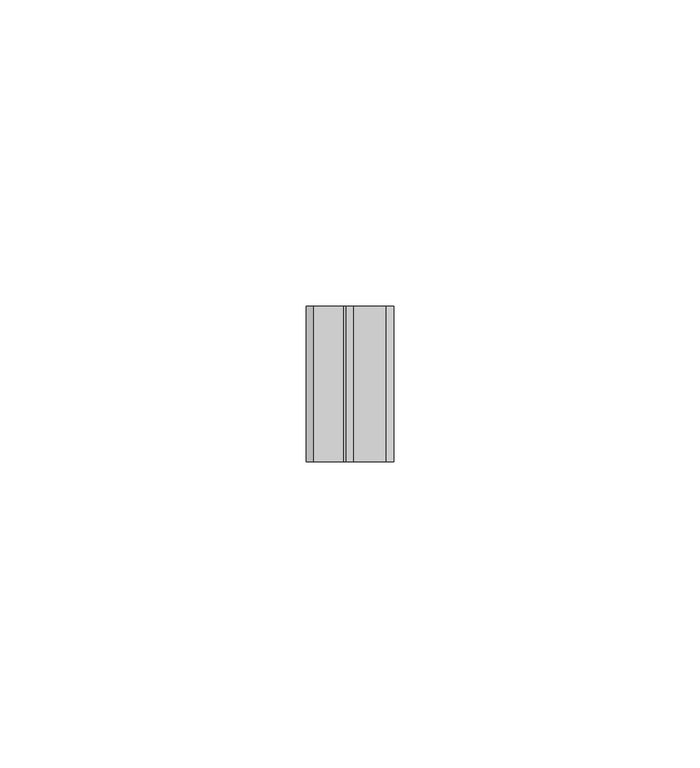
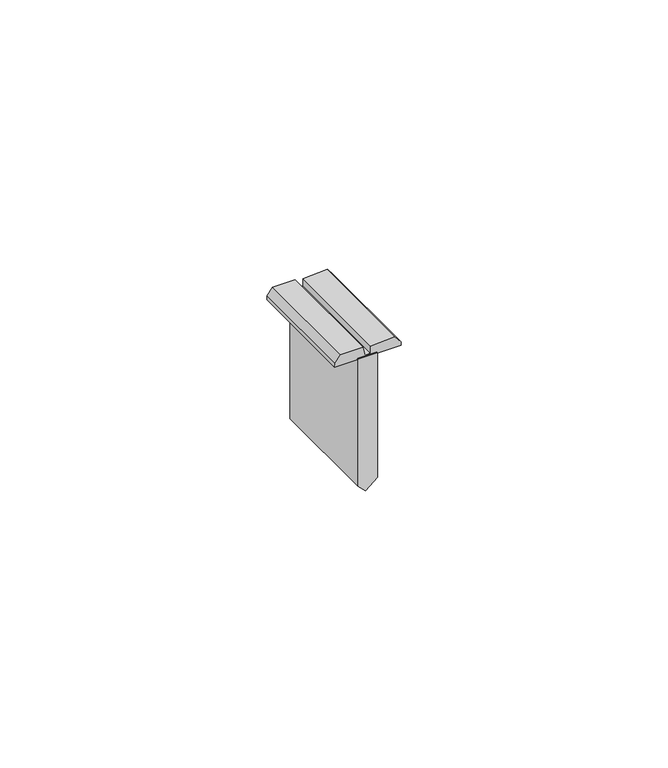
"""IFC4 building model written with IfcOpenShell, lengths in millimetres: proxy geometry, FASTENER005 5969 : FASTENER005 5969."""

import ifcopenshell
import ifcopenshell.guid

model = None  # the IFC model being written
_history = None  # IfcOwnerHistory: only IFC2X3 demands one
_inside = {}  # id of a spatial element -> (the spatial element, [elements in it])
_under = {}  # id of a project, library or spatial element -> (it, [spatial elements below it])
_declared = {}  # id of a project -> (the project, [libraries it declares])
_typed = {}  # id of a type object -> (the type object, [elements of that type])
_made_of = {}  # id of a material, layer set ... -> (it, [elements and type objects made of it])


def new_model(schema):
    """Start an empty IFC model of exactly this schema.

    Asked for "IFC4X3", IfcOpenShell would pick the latest addendum, in which some entities
    have other attributes; the version numbers below select the first issue.
    IFC2X3 requires an IfcOwnerHistory on every rooted entity: one is made here for all.
    """
    global model, _history
    if schema == "IFC4X3":
        model = ifcopenshell.file(schema_version=(4, 3, 0, 0))
    else:
        model = ifcopenshell.file(schema=schema)
    _inside.clear()
    _under.clear()
    _declared.clear()
    _typed.clear()
    _made_of.clear()
    _history = None
    if model.schema == "IFC2X3":
        org = make("IfcOrganization", Name="unknown")
        user = make(
            "IfcPersonAndOrganization",
            ThePerson=make("IfcPerson", FamilyName="unknown"),
            TheOrganization=org,
        )
        app = make(
            "IfcApplication",
            ApplicationDeveloper=org,
            Version="unknown",
            ApplicationFullName="unknown",
            ApplicationIdentifier="unknown",
        )
        _history = make(
            "IfcOwnerHistory",
            OwningUser=user,
            OwningApplication=app,
            ChangeAction="ADDED",
            CreationDate=0,
        )
    return model


def make(cls, **values):
    """One entity of the class cls with the attributes given. An attribute that is None is left unset."""
    return model.create_entity(
        cls, **{name: value for name, value in values.items() if value is not None}
    )


def rooted(cls, **values):
    """An entity with a GlobalId (a new one), such as an element, a storey or a relation."""
    return make(cls, GlobalId=ifcopenshell.guid.new(), OwnerHistory=_history, **values)


def si_unit(unit_type, name, prefix=None):
    """IfcSIUnit, for example si_unit("LENGTHUNIT", "METRE", prefix="MILLI")."""
    return make("IfcSIUnit", UnitType=unit_type, Prefix=prefix, Name=name)


def assignment(units):
    """IfcUnitAssignment: the units of a project."""
    return None if units is None else make("IfcUnitAssignment", Units=units)


def point(xyz):
    """IfcCartesianPoint."""
    return None if xyz is None else make("IfcCartesianPoint", Coordinates=xyz)


def direction(xyz):
    """IfcDirection."""
    return None if xyz is None else make("IfcDirection", DirectionRatios=xyz)


def frame(location, z_axis=None, x_axis=None):
    """IfcAxis2Placement3D, a coordinate frame: its origin and axes. An axis left out is left unset."""
    return make(
        "IfcAxis2Placement3D",
        Location=point(location),
        Axis=direction(z_axis),
        RefDirection=direction(x_axis),
    )


def origin():
    """The frame at (0, 0, 0) with its axes left unset."""
    return frame((0.0, 0.0, 0.0))


def place(relative_to, where):
    """IfcLocalPlacement: puts the frame where relative to a parent placement (None: the world)."""
    return make(
        "IfcLocalPlacement", PlacementRelTo=relative_to, RelativePlacement=where
    )


def context(
    kind, dimensions, precision=None, world=None, true_north=None, identifier=None
):
    """IfcGeometricRepresentationContext, for example the 3D "Model" context."""
    return make(
        "IfcGeometricRepresentationContext",
        ContextIdentifier=identifier,
        ContextType=kind,
        CoordinateSpaceDimension=dimensions,
        Precision=precision,
        WorldCoordinateSystem=world,
        TrueNorth=true_north,
    )


def project(units=None, contexts=None):
    """IfcProject with its units and contexts."""
    return rooted(
        "IfcProject",
        Name="project",
        RepresentationContexts=contexts,
        UnitsInContext=assignment(units),
    )


def spatial(cls, under=None, at=None, **own):
    """A site, building, storey or space (cls), placed at a placement, below another one or the project."""
    s = rooted(cls, ObjectPlacement=at, **own)
    if under is not None:
        _under.setdefault(under.id(), (under, []))[1].append(s)
    return s


def polyline(points):
    """IfcPolyline through the points."""
    return make("IfcPolyline", Points=[point(p) for p in points])


def outline(outer, holes=None, kind="AREA"):
    """IfcArbitraryClosedProfileDef: a profile drawn as a closed curve; with holes, ...WithVoids."""
    if holes is None:
        return make("IfcArbitraryClosedProfileDef", ProfileType=kind, OuterCurve=outer)
    return make(
        "IfcArbitraryProfileDefWithVoids",
        ProfileType=kind,
        OuterCurve=outer,
        InnerCurves=holes,
    )


def extrude(swept, where, along, depth):
    """IfcExtrudedAreaSolid: the profile swept, set in the frame where, extruded along a direction by depth."""
    return make(
        "IfcExtrudedAreaSolid",
        SweptArea=swept,
        Position=where,
        ExtrudedDirection=direction(along),
        Depth=depth,
    )


def shape(context_of_items, identifier, shape_type, items):
    """IfcShapeRepresentation: the items that make up one representation, for example the "Body"."""
    return make(
        "IfcShapeRepresentation",
        ContextOfItems=context_of_items,
        RepresentationIdentifier=identifier,
        RepresentationType=shape_type,
        Items=items,
    )


def source(mapping_origin, context_of_items, identifier, shape_type, items):
    """IfcRepresentationMap: a shape defined once, which mapped items show again and again."""
    return make(
        "IfcRepresentationMap",
        MappingOrigin=mapping_origin,
        MappedRepresentation=shape(context_of_items, identifier, shape_type, items),
    )


def transform(
    local_origin,
    x_axis=None,
    y_axis=None,
    z_axis=None,
    scale=None,
    scale2=None,
    scale3=None,
    uniform=True,
):
    """IfcCartesianTransformationOperator3D, or its non-uniform kind. x_axis, y_axis, z_axis: its Axis1, 2, 3."""
    if uniform:
        return make(
            "IfcCartesianTransformationOperator3D",
            Axis1=direction(x_axis),
            Axis2=direction(y_axis),
            LocalOrigin=point(local_origin),
            Scale=scale,
            Axis3=direction(z_axis),
        )
    return make(
        "IfcCartesianTransformationOperator3DnonUniform",
        Axis1=direction(x_axis),
        Axis2=direction(y_axis),
        LocalOrigin=point(local_origin),
        Scale=scale,
        Axis3=direction(z_axis),
        Scale2=scale2,
        Scale3=scale3,
    )


def mapped(mapping_source, mapping_target):
    """IfcMappedItem: shows the shape of a source again, moved by a transform."""
    return make(
        "IfcMappedItem", MappingSource=mapping_source, MappingTarget=mapping_target
    )


def made_of(thing, what):
    """Note that an element or type object is made of a material, layer set ...; save() writes the relation."""
    if what is not None:
        _made_of.setdefault(what.id(), (what, []))[1].append(thing)
    return thing


def element(
    cls,
    number,
    at=None,
    inside=None,
    cuts=None,
    type_object=None,
    material=None,
    context=None,
    identifier="Body",
    shape_type=None,
    held_by="IfcProductDefinitionShape",
    body=None,
    shapes=None,
    **own,
):
    """One element of the class cls, such as IfcWall. Its Tag is "e" and its number.

    at: its placement. inside: the storey or other place that contains it. cuts: it is an
    opening in that element (IfcRelVoidsElement). A single representation is given by context,
    identifier, shape_type and body (its items); several are given by shapes. held_by: the class
    of the entity that holds the representations. save() writes the other relations.
    """
    e = rooted(cls, Tag="e%d" % number, ObjectPlacement=at, **own)
    if body is not None:
        shapes = [shape(context, identifier, shape_type, body)]
    if shapes is not None:
        e.Representation = make(held_by, Representations=shapes)
    if inside is not None:
        _inside.setdefault(inside.id(), (inside, []))[1].append(e)
    if cuts is not None:
        rooted(
            "IfcRelVoidsElement", RelatingBuildingElement=cuts, RelatedOpeningElement=e
        )
    if type_object is not None:
        _typed.setdefault(type_object.id(), (type_object, []))[1].append(e)
    return made_of(e, material)


def aggregate(whole, parts):
    """IfcRelAggregates: a whole, such as a stair, and the parts it consists of."""
    return rooted("IfcRelAggregates", RelatingObject=whole, RelatedObjects=parts)


def save(model, path):
    """Write the relations noted so far, then the file.

    IfcRelAggregates (storeys below a building ...), IfcRelContainedInSpatialStructure (elements
    in a storey), IfcRelDefinesByType, IfcRelAssociatesMaterial and IfcRelDeclares: one each for
    every whole, place, type object, material and project.
    """
    for whole, parts in _under.values():
        aggregate(whole, parts)
    for where, things in _inside.values():
        rooted(
            "IfcRelContainedInSpatialStructure",
            RelatedElements=things,
            RelatingStructure=where,
        )
    for kind, things in _typed.values():
        rooted("IfcRelDefinesByType", RelatedObjects=things, RelatingType=kind)
    for what, things in _made_of.values():
        rooted("IfcRelAssociatesMaterial", RelatedObjects=things, RelatingMaterial=what)
    for by, libraries in _declared.values():
        rooted("IfcRelDeclares", RelatingContext=by, RelatedDefinitions=libraries)
    model.write(path)


def generic_models_4a0cef2c(model_context):
    return source(origin(), model_context, "Body", "SweptSolid", [
        extrude(outline(polyline([(42579.6987049, 5977.3107075), (42550.7399648, 5977.3107075), (42549.1244121, 5978.9677221), (42551.3049701, 5981.517626), (42579.6987049, 5981.517626), (42579.6987049, 5977.3107075)])), frame((0.0, -1078.2906574, 0.0), z_axis=(0.0, 1.0, 0.0), x_axis=(0.0, 0.0, 1.0)), (0.0, 0.0, 1.0), 25.4),
        extrude(outline(polyline([(42579.6987049, 5986.5634932), (42580.508527, 5986.5634932), (42582.1023984, 5985.3247911), (42581.7061629, 5980.0391089), (42580.1167322, 5980.0391089), (42580.1167322, 5978.792004), (42582.1288635, 5978.3957685), (42582.1288635, 5973.5166866), (42580.5349921, 5972.2779845), (42579.6987049, 5972.2671879), (42579.6987049, 5986.5634932)])), frame((0.0, -1078.2906574, 0.0), z_axis=(0.0, 1.0, 0.0), x_axis=(0.0, 0.0, 1.0)), (0.0, 0.0, 1.0), 25.4),
    ])


if __name__ == "__main__":
    model = new_model("IFC4")
    model_context = context("Model", 3, world=origin())
    ifc_project = project(units=[si_unit("LENGTHUNIT", "METRE", prefix="MILLI")], contexts=[model_context])
    site = spatial("IfcSite", under=ifc_project)
    building = spatial("IfcBuilding", under=site)
    placement = place(None, origin())
    generic_models_shape = generic_models_4a0cef2c(model_context)
    element("IfcBuildingElementProxy", 1, Name="FASTENER005 5969 : FASTENER005 5969", ObjectType="FASTENER005 5969 : FASTENER005 5969", at=placement, inside=building, context=model_context, shape_type="MappedRepresentation", body=[
        mapped(generic_models_shape, transform((0.0, 0.0, 0.0), x_axis=(1.0, 0.0, 0.0), y_axis=(0.0, 1.0, 0.0), z_axis=(0.0, 0.0, 1.0))),
    ])
    save(model, "model.ifc")

# Revit data of these elements
# Type "FASTENER005 5969 : FASTENER005 5969"
#   NameOverride = "FASTENER005"
# Element 1 (IfcBuildingElementProxy, "FASTENER005 5969 : FASTENER005 5969")
#   Materials on its faces: "ENGINEERED PANCAKE HEAD FASTENER (NOT BY AEP-SPAN) @ 12\" O.C."
# Materials
#   "ENGINEERED PANCAKE HEAD FASTENER (NOT BY AEP-SPAN) @ 12\" O.C.": class "Unassigned", colour RGB 255 255 255, transparency 0
